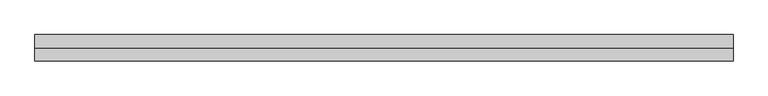
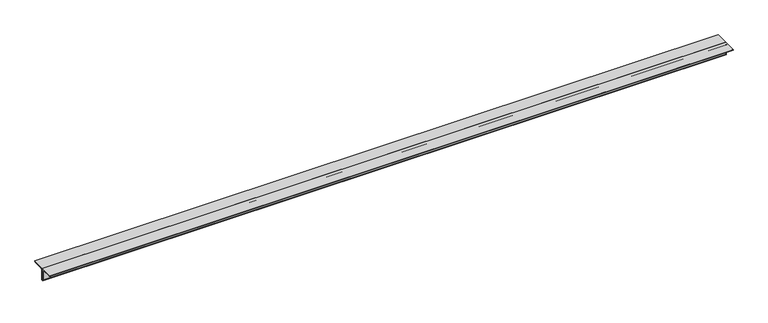
"""IFC4 building model written with IfcOpenShell, lengths in millimetres: member geometry, Steel Framing_2Ls_KS : H_SB_AR_S02_2Ls-100x100x10_VBR1."""

from ifc_helpers import new_model, si_unit, point, frame, frame_2d, origin, place, context, project, spatial, polyline, circle_curve, trimmed, segment, composite_curve, outline, extrude, source, transform, mapped, element, save


def member_7b01582b(model_context):
    return source(origin(), model_context, "Body", "SweptSolid", [
        extrude(outline(composite_curve([segment(polyline([(0.0, 28.2), (100.0, 28.2)]), True, "CONTINUOUS"), segment(trimmed(circle_curve(frame_2d((90.0, 28.2)), 10.0), [point((100.0, 28.2))], [point((90.0, 18.2))], False, "CARTESIAN"), True, "CONTINUOUS"), segment(polyline([(90.0, 18.2), (20.0, 18.2)]), True, "CONTINUOUS"), segment(trimmed(circle_curve(frame_2d((20.0, 8.2)), 10.0), [point((20.0, 18.2))], [point((10.0, 8.2))], True, "CARTESIAN"), True, "CONTINUOUS"), segment(polyline([(10.0, 8.2), (10.0, -61.8)]), True, "CONTINUOUS"), segment(trimmed(circle_curve(frame_2d((0.0, -61.8)), 10.0), [point((10.0, -61.8))], [point((0.0, -71.8))], False, "CARTESIAN"), True, "CONTINUOUS"), segment(polyline([(0.0, -71.8), (0.0, 28.2)]), True, "CONTINUOUS")], self_intersect=False)), frame((-2838.463978, 0.0, 0.0), z_axis=(1.0, 0.0, 0.0), x_axis=(0.0, 1.0, 0.0)), (0.0, 0.0, 1.0), 5283.025664),
        extrude(outline(composite_curve([segment(polyline([(0.0, 28.2), (0.0, -71.8)]), True, "CONTINUOUS"), segment(trimmed(circle_curve(frame_2d((0.0, -61.8)), 10.0), [point((0.0, -71.8))], [point((-10.0, -61.8))], False, "CARTESIAN"), True, "CONTINUOUS"), segment(polyline([(-10.0, -61.8), (-10.0, 8.2)]), True, "CONTINUOUS"), segment(trimmed(circle_curve(frame_2d((-20.0, 8.2)), 10.0), [point((-10.0, 8.2))], [point((-20.0, 18.2))], True, "CARTESIAN"), True, "CONTINUOUS"), segment(polyline([(-20.0, 18.2), (-90.0, 18.2)]), True, "CONTINUOUS"), segment(trimmed(circle_curve(frame_2d((-90.0, 28.2)), 10.0), [point((-90.0, 18.2))], [point((-100.0, 28.2))], False, "CARTESIAN"), True, "CONTINUOUS"), segment(polyline([(-100.0, 28.2), (0.0, 28.2)]), True, "CONTINUOUS")], self_intersect=False)), frame((-2838.463978, 0.0, 0.0), z_axis=(1.0, 0.0, 0.0), x_axis=(0.0, 1.0, 0.0)), (0.0, 0.0, 1.0), 5283.025664),
    ])


if __name__ == "__main__":
    model = new_model("IFC4")
    model_context = context("Model", 3, world=origin())
    ifc_project = project(units=[si_unit("LENGTHUNIT", "METRE", prefix="MILLI")], contexts=[model_context])
    site = spatial("IfcSite", under=ifc_project)
    building = spatial("IfcBuilding", under=site)
    placement = place(None, origin())
    member_shape = member_7b01582b(model_context)
    element("IfcMember", 1, ObjectType="Steel Framing_2Ls_KS : H_SB_AR_S02_2Ls-100x100x10_VBR1", at=placement, inside=building, context=model_context, shape_type="MappedRepresentation", body=[
        mapped(member_shape, transform((0.0, 0.0, 0.0), x_axis=(1.0, 0.0, 0.0), y_axis=(0.0, 1.0, 0.0), z_axis=(0.0, 0.0, 1.0))),
    ])
    save(model, "model.ifc")

# Revit data of these elements
# Type "Steel Framing_2Ls_KS : H_SB_AR_S02_2Ls-100x100x10_VBR1"
#   Type Comments = "MAIN"
#   Type Mark = "VBR1"
#   H_SectionID = "2Ls-100x100x10"
#   Assembly Code = "B10"
#   Legs = "LLBB"
#   H_Ratio for Additional Steel Plate = 0.2
#   W = 0
#   Perimeter = 0.80 m²/m
#   Nominal Weight = 29.80 kgf/m
#   Length [instance default] = 1524 mm
#   Space = 0 mm
#   b = 100 mm
#   d = 100 mm
#   t = 10 mm
#   y = 28.2 mm
#   A = 0.0038 m²
#   Structural Material [instance default] = Steel, 45-345
# Element 1 (IfcMember, "Steel Framing_2Ls_KS : H_SB_AR_S02_2Ls-100x100x10_VBR1")
#   Materials on its faces: "Steel, 45-345"
# Materials
#   "Steel, 45-345": class "Metal", colour RGB 189 187 185, transparency 0, Description = "Steel 345 MPa", Cost = 0
